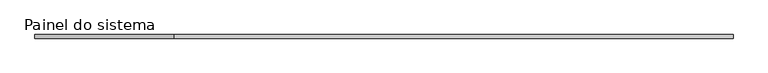
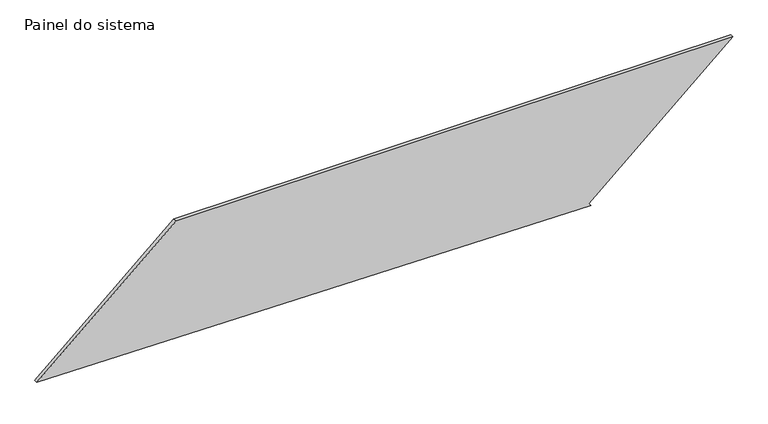
"""IFC4 building model written with IfcOpenShell, lengths in millimetres: plate geometry, Painel do sistema : Envidraçado."""

from ifc_helpers import new_model, si_unit, frame, origin, place, context, project, spatial, polyline, outline, extrude, source, transform, mapped, element, save


def painel_do_sistema_e3f3e6a8(model_context):
    return source(origin(), model_context, "Body", "SweptSolid", [
        extrude(outline(polyline([(0.0, 1432.8353221), (18.8079041, 1416.3652661), (894.4054699, 2416.2498538), (894.4054699, -1450.8119292), (48.9727998, -2416.2498538), (0.0, 1432.8353221)])), frame((0.0, 24.5, 0.0), z_axis=(0.0, 1.0, 0.0), x_axis=(0.0, 0.0, 1.0)), (0.0, 0.0, 1.0), 25.0),
    ])


if __name__ == "__main__":
    model = new_model("IFC4")
    model_context = context("Model", 3, world=origin())
    ifc_project = project(units=[si_unit("LENGTHUNIT", "METRE", prefix="MILLI")], contexts=[model_context])
    site = spatial("IfcSite", under=ifc_project)
    building = spatial("IfcBuilding", under=site)
    placement = place(None, origin())
    painel_do_sistema_shape = painel_do_sistema_e3f3e6a8(model_context)
    element("IfcPlate", 1, ObjectType="Painel do sistema : Envidraçado", at=placement, inside=building, context=model_context, shape_type="MappedRepresentation", body=[
        mapped(painel_do_sistema_shape, transform((0.0, 0.0, 0.0), x_axis=(1.0, 0.0, 0.0), y_axis=(0.0, 1.0, 0.0), z_axis=(0.0, 0.0, 1.0))),
    ])
    save(model, "model.ifc")

# Revit data of these elements
# Type "Painel do sistema : Envidraçado"
#   Construction Type Id = "GSP4R"
#   Analytic Construction = "Vidraça única Pilkington 1/8 pol"
#   Visual Light Transmittance = 0.9
#   Solar Heat Gain Coefficient = 0.86
#   Heat Transfer Coefficient (U) = 6.7069 W/(m²·K)
# Element 1 (IfcPlate, "Painel do sistema : Envidraçado")
#   Materials on its faces: "Vidro"
# Materials
#   "Vidro": class "Vidro", colour RGB 0 128 192, transparency 0.9, Description = "Vidro de sílica", Cost = 0
